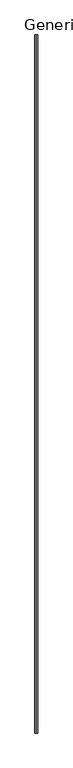
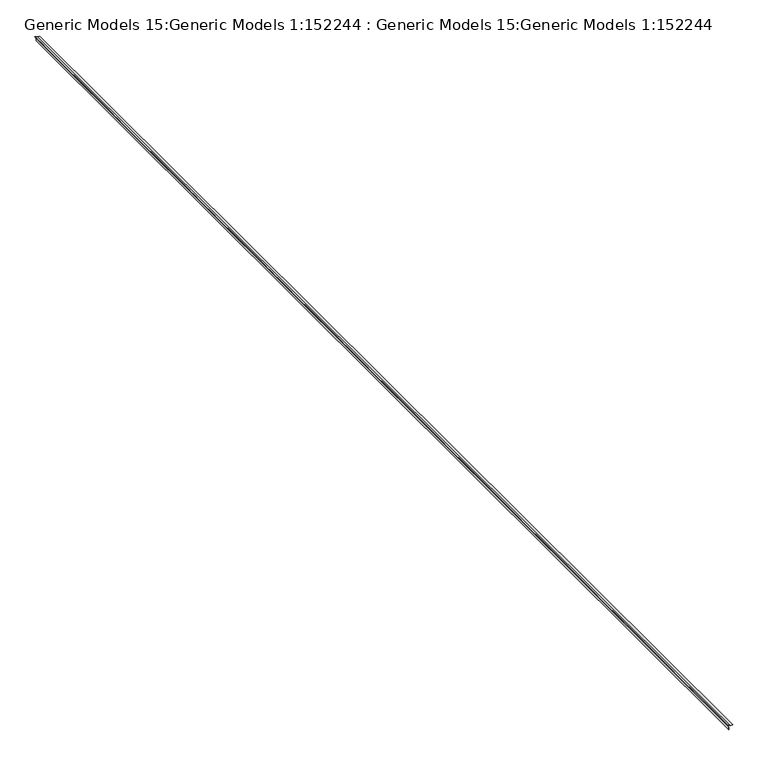
"""IFC4 building model written with IfcOpenShell, lengths in millimetres: proxy geometry, Generic Models 15:Generic Models 1:152244 : Generic Models 15:Generic Models 1:152244."""

import ifcopenshell
import ifcopenshell.guid

model = None  # the IFC model being written
_history = None  # IfcOwnerHistory: only IFC2X3 demands one
_inside = {}  # id of a spatial element -> (the spatial element, [elements in it])
_under = {}  # id of a project, library or spatial element -> (it, [spatial elements below it])
_declared = {}  # id of a project -> (the project, [libraries it declares])
_typed = {}  # id of a type object -> (the type object, [elements of that type])
_made_of = {}  # id of a material, layer set ... -> (it, [elements and type objects made of it])


def new_model(schema):
    """Start an empty IFC model of exactly this schema.

    Asked for "IFC4X3", IfcOpenShell would pick the latest addendum, in which some entities
    have other attributes; the version numbers below select the first issue.
    IFC2X3 requires an IfcOwnerHistory on every rooted entity: one is made here for all.
    """
    global model, _history
    if schema == "IFC4X3":
        model = ifcopenshell.file(schema_version=(4, 3, 0, 0))
    else:
        model = ifcopenshell.file(schema=schema)
    _inside.clear()
    _under.clear()
    _declared.clear()
    _typed.clear()
    _made_of.clear()
    _history = None
    if model.schema == "IFC2X3":
        org = make("IfcOrganization", Name="unknown")
        user = make(
            "IfcPersonAndOrganization",
            ThePerson=make("IfcPerson", FamilyName="unknown"),
            TheOrganization=org,
        )
        app = make(
            "IfcApplication",
            ApplicationDeveloper=org,
            Version="unknown",
            ApplicationFullName="unknown",
            ApplicationIdentifier="unknown",
        )
        _history = make(
            "IfcOwnerHistory",
            OwningUser=user,
            OwningApplication=app,
            ChangeAction="ADDED",
            CreationDate=0,
        )
    return model


def make(cls, **values):
    """One entity of the class cls with the attributes given. An attribute that is None is left unset."""
    return model.create_entity(
        cls, **{name: value for name, value in values.items() if value is not None}
    )


def rooted(cls, **values):
    """An entity with a GlobalId (a new one), such as an element, a storey or a relation."""
    return make(cls, GlobalId=ifcopenshell.guid.new(), OwnerHistory=_history, **values)


def si_unit(unit_type, name, prefix=None):
    """IfcSIUnit, for example si_unit("LENGTHUNIT", "METRE", prefix="MILLI")."""
    return make("IfcSIUnit", UnitType=unit_type, Prefix=prefix, Name=name)


def assignment(units):
    """IfcUnitAssignment: the units of a project."""
    return None if units is None else make("IfcUnitAssignment", Units=units)


def point(xyz):
    """IfcCartesianPoint."""
    return None if xyz is None else make("IfcCartesianPoint", Coordinates=xyz)


def direction(xyz):
    """IfcDirection."""
    return None if xyz is None else make("IfcDirection", DirectionRatios=xyz)


def frame(location, z_axis=None, x_axis=None):
    """IfcAxis2Placement3D, a coordinate frame: its origin and axes. An axis left out is left unset."""
    return make(
        "IfcAxis2Placement3D",
        Location=point(location),
        Axis=direction(z_axis),
        RefDirection=direction(x_axis),
    )


def frame_2d(location, x_axis=None):
    """IfcAxis2Placement2D, a coordinate frame in the plane: its origin and x axis."""
    return make(
        "IfcAxis2Placement2D", Location=point(location), RefDirection=direction(x_axis)
    )


def origin():
    """The frame at (0, 0, 0) with its axes left unset."""
    return frame((0.0, 0.0, 0.0))


def place(relative_to, where):
    """IfcLocalPlacement: puts the frame where relative to a parent placement (None: the world)."""
    return make(
        "IfcLocalPlacement", PlacementRelTo=relative_to, RelativePlacement=where
    )


def context(
    kind, dimensions, precision=None, world=None, true_north=None, identifier=None
):
    """IfcGeometricRepresentationContext, for example the 3D "Model" context."""
    return make(
        "IfcGeometricRepresentationContext",
        ContextIdentifier=identifier,
        ContextType=kind,
        CoordinateSpaceDimension=dimensions,
        Precision=precision,
        WorldCoordinateSystem=world,
        TrueNorth=true_north,
    )


def project(units=None, contexts=None):
    """IfcProject with its units and contexts."""
    return rooted(
        "IfcProject",
        Name="project",
        RepresentationContexts=contexts,
        UnitsInContext=assignment(units),
    )


def spatial(cls, under=None, at=None, **own):
    """A site, building, storey or space (cls), placed at a placement, below another one or the project."""
    s = rooted(cls, ObjectPlacement=at, **own)
    if under is not None:
        _under.setdefault(under.id(), (under, []))[1].append(s)
    return s


def polyline(points):
    """IfcPolyline through the points."""
    return make("IfcPolyline", Points=[point(p) for p in points])


def circle_curve(where, radius):
    """IfcCircle in the frame where."""
    return make("IfcCircle", Position=where, Radius=radius)


def trimmed(basis, trim1, trim2, sense, master):
    """IfcTrimmedCurve: the piece of a basis curve between two trims."""
    return make(
        "IfcTrimmedCurve",
        BasisCurve=basis,
        Trim1=trim1,
        Trim2=trim2,
        SenseAgreement=sense,
        MasterRepresentation=master,
    )


def segment(curve, same_sense, transition):
    """IfcCompositeCurveSegment."""
    return make(
        "IfcCompositeCurveSegment",
        Transition=transition,
        SameSense=same_sense,
        ParentCurve=curve,
    )


def composite_curve(segments, self_intersect=None):
    """IfcCompositeCurve: segments joined end to end."""
    return make("IfcCompositeCurve", Segments=segments, SelfIntersect=self_intersect)


def outline(outer, holes=None, kind="AREA"):
    """IfcArbitraryClosedProfileDef: a profile drawn as a closed curve; with holes, ...WithVoids."""
    if holes is None:
        return make("IfcArbitraryClosedProfileDef", ProfileType=kind, OuterCurve=outer)
    return make(
        "IfcArbitraryProfileDefWithVoids",
        ProfileType=kind,
        OuterCurve=outer,
        InnerCurves=holes,
    )


def extrude(swept, where, along, depth):
    """IfcExtrudedAreaSolid: the profile swept, set in the frame where, extruded along a direction by depth."""
    return make(
        "IfcExtrudedAreaSolid",
        SweptArea=swept,
        Position=where,
        ExtrudedDirection=direction(along),
        Depth=depth,
    )


def shape(context_of_items, identifier, shape_type, items):
    """IfcShapeRepresentation: the items that make up one representation, for example the "Body"."""
    return make(
        "IfcShapeRepresentation",
        ContextOfItems=context_of_items,
        RepresentationIdentifier=identifier,
        RepresentationType=shape_type,
        Items=items,
    )


def source(mapping_origin, context_of_items, identifier, shape_type, items):
    """IfcRepresentationMap: a shape defined once, which mapped items show again and again."""
    return make(
        "IfcRepresentationMap",
        MappingOrigin=mapping_origin,
        MappedRepresentation=shape(context_of_items, identifier, shape_type, items),
    )


def transform(
    local_origin,
    x_axis=None,
    y_axis=None,
    z_axis=None,
    scale=None,
    scale2=None,
    scale3=None,
    uniform=True,
):
    """IfcCartesianTransformationOperator3D, or its non-uniform kind. x_axis, y_axis, z_axis: its Axis1, 2, 3."""
    if uniform:
        return make(
            "IfcCartesianTransformationOperator3D",
            Axis1=direction(x_axis),
            Axis2=direction(y_axis),
            LocalOrigin=point(local_origin),
            Scale=scale,
            Axis3=direction(z_axis),
        )
    return make(
        "IfcCartesianTransformationOperator3DnonUniform",
        Axis1=direction(x_axis),
        Axis2=direction(y_axis),
        LocalOrigin=point(local_origin),
        Scale=scale,
        Axis3=direction(z_axis),
        Scale2=scale2,
        Scale3=scale3,
    )


def mapped(mapping_source, mapping_target):
    """IfcMappedItem: shows the shape of a source again, moved by a transform."""
    return make(
        "IfcMappedItem", MappingSource=mapping_source, MappingTarget=mapping_target
    )


def made_of(thing, what):
    """Note that an element or type object is made of a material, layer set ...; save() writes the relation."""
    if what is not None:
        _made_of.setdefault(what.id(), (what, []))[1].append(thing)
    return thing


def element(
    cls,
    number,
    at=None,
    inside=None,
    cuts=None,
    type_object=None,
    material=None,
    context=None,
    identifier="Body",
    shape_type=None,
    held_by="IfcProductDefinitionShape",
    body=None,
    shapes=None,
    **own,
):
    """One element of the class cls, such as IfcWall. Its Tag is "e" and its number.

    at: its placement. inside: the storey or other place that contains it. cuts: it is an
    opening in that element (IfcRelVoidsElement). A single representation is given by context,
    identifier, shape_type and body (its items); several are given by shapes. held_by: the class
    of the entity that holds the representations. save() writes the other relations.
    """
    e = rooted(cls, Tag="e%d" % number, ObjectPlacement=at, **own)
    if body is not None:
        shapes = [shape(context, identifier, shape_type, body)]
    if shapes is not None:
        e.Representation = make(held_by, Representations=shapes)
    if inside is not None:
        _inside.setdefault(inside.id(), (inside, []))[1].append(e)
    if cuts is not None:
        rooted(
            "IfcRelVoidsElement", RelatingBuildingElement=cuts, RelatedOpeningElement=e
        )
    if type_object is not None:
        _typed.setdefault(type_object.id(), (type_object, []))[1].append(e)
    return made_of(e, material)


def aggregate(whole, parts):
    """IfcRelAggregates: a whole, such as a stair, and the parts it consists of."""
    return rooted("IfcRelAggregates", RelatingObject=whole, RelatedObjects=parts)


def save(model, path):
    """Write the relations noted so far, then the file.

    IfcRelAggregates (storeys below a building ...), IfcRelContainedInSpatialStructure (elements
    in a storey), IfcRelDefinesByType, IfcRelAssociatesMaterial and IfcRelDeclares: one each for
    every whole, place, type object, material and project.
    """
    for whole, parts in _under.values():
        aggregate(whole, parts)
    for where, things in _inside.values():
        rooted(
            "IfcRelContainedInSpatialStructure",
            RelatedElements=things,
            RelatingStructure=where,
        )
    for kind, things in _typed.values():
        rooted("IfcRelDefinesByType", RelatedObjects=things, RelatingType=kind)
    for what, things in _made_of.values():
        rooted("IfcRelAssociatesMaterial", RelatedObjects=things, RelatingMaterial=what)
    for by, libraries in _declared.values():
        rooted("IfcRelDeclares", RelatingContext=by, RelatedDefinitions=libraries)
    model.write(path)


def generic_models_15_generic_models_1_152244_generic_models_15_03b073f8(model_context):
    return source(origin(), model_context, "Body", "SweptSolid", [
        extrude(outline(composite_curve([segment(polyline([(3637.915, -9462.7819046), (3657.4416156, -9500.8074192)]), True, "CONTINUOUS"), segment(trimmed(circle_curve(frame_2d((3656.1657873, -9501.4625743)), 1.4342127), [point((3657.4416156, -9500.8074192))], [point((3655.5106323, -9502.7384026))], False, "CARTESIAN"), True, "CONTINUOUS"), segment(polyline([(3655.5106323, -9502.7384026), (3617.4851176, -9483.211787), (3579.3851176, -9483.211787), (3579.3851176, -9481.941787), (3617.7921414, -9481.941787), (3656.5452396, -9501.8420266), (3636.645, -9463.0889283), (3636.645, -9424.6819046), (3637.915, -9424.6819046), (3637.915, -9462.7819046)]), True, "CONTINUOUS")], self_intersect=False)), frame((0.0, -6877.9974793, 0.0), z_axis=(0.0, 1.0, 0.0), x_axis=(0.0, 0.0, 1.0)), (0.0, 0.0, 1.0), 19050.0),
    ])


if __name__ == "__main__":
    model = new_model("IFC4")
    model_context = context("Model", 3, world=origin())
    ifc_project = project(units=[si_unit("LENGTHUNIT", "METRE", prefix="MILLI")], contexts=[model_context])
    site = spatial("IfcSite", under=ifc_project)
    building = spatial("IfcBuilding", under=site)
    placement = place(None, origin())
    generic_models_15_generic_models_1_152244_generic_models_15_shape = generic_models_15_generic_models_1_152244_generic_models_15_03b073f8(model_context)
    element("IfcBuildingElementProxy", 1, Name="Generic Models 15:Generic Models 1:152244 : Generic Models 15:Generic Models 1:152244", ObjectType="Generic Models 15:Generic Models 1:152244 : Generic Models 15:Generic Models 1:152244", at=placement, inside=building, context=model_context, shape_type="MappedRepresentation", body=[
        mapped(generic_models_15_generic_models_1_152244_generic_models_15_shape, transform((0.0, 0.0, 0.0), x_axis=(1.0, 0.0, 0.0), y_axis=(0.0, 1.0, 0.0), z_axis=(0.0, 0.0, 1.0))),
    ])
    save(model, "model.ifc")

# Revit data of these elements
# Type "Generic Models 15:Generic Models 1:152244 : Generic Models 15:Generic Models 1:152244"
#   NameOverride = "Generic Models 15:Generic Models 1:152244"
#   ObjectTypeOverride = "Generic Models 15:Generic Models 1"
#   Reference = "Generic Models 1"
#   Category = "Generic Models"
#   Tag = "152244"
# Element 1 (IfcBuildingElementProxy, "Generic Models 15:Generic Models 1:152244 : Generic Models 15:Generic Models 1:152244")
#   Materials on its faces: "_CONTINUOUS 16 GA. COPPER CORNER BEAD 558"
# Materials
#   "_CONTINUOUS 16 GA. COPPER CORNER BEAD 558": class "Unassigned", colour RGB 253 192 103, transparency 0
